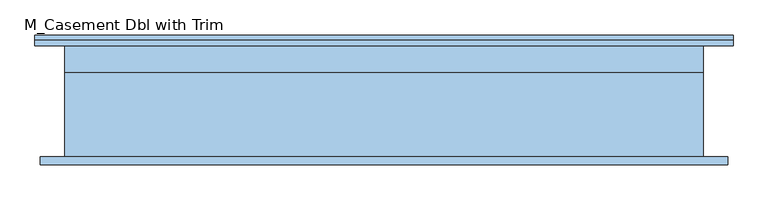
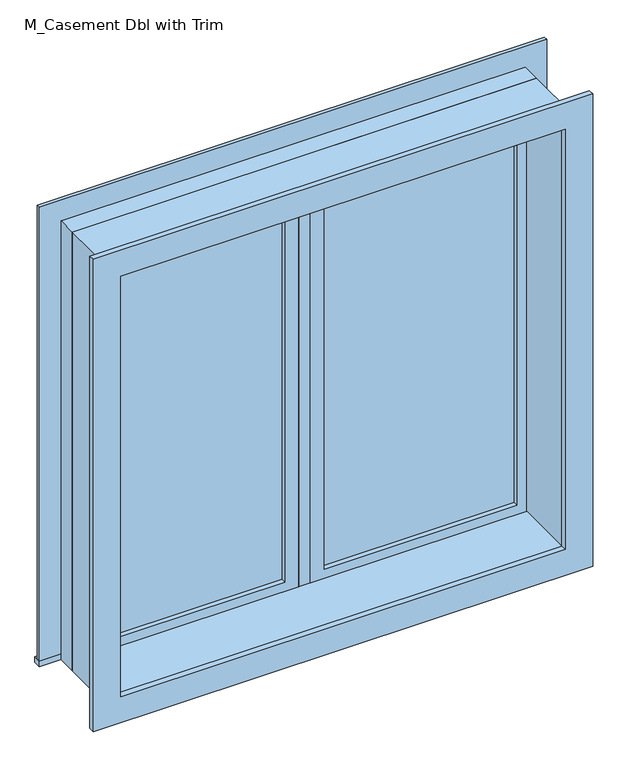
"""IFC4 building model written with IfcOpenShell, lengths in millimetres: window geometry, M_Casement Dbl with Trim : 150x150cm Pencere."""

from ifc_helpers import new_model, si_unit, frame, origin, place, context, project, spatial, polyline, outline, extrude, source, transform, mapped, element, save


def m_casement_dbl_with_trim_011da180(model_context):
    return source(origin(), model_context, "Body", "SweptSolid", [
        extrude(outline(polyline([(63.5, 114.175), (686.5, 114.175), (686.5, 101.475), (63.5, 101.475), (63.5, 114.175)])), frame((0.0, 0.0, 978.5), z_axis=(0.0, 0.0, 1.0), x_axis=(1.0, 0.0, 0.0)), (0.0, 0.0, 1.0), 1373.0),
        extrude(outline(polyline([(2395.95, 19.05), (934.05, 19.05), (934.05, 730.95), (2395.95, 730.95), (2395.95, 19.05)]), holes=[polyline([(2351.5, 63.5), (2351.5, 686.5), (978.5, 686.5), (978.5, 63.5), (2351.5, 63.5)])]), frame((0.0, 85.6, 0.0), z_axis=(0.0, 1.0, 0.0), x_axis=(0.0, 0.0, 1.0)), (0.0, 0.0, 1.0), 44.45),
        extrude(outline(polyline([(-819.95, 174.75), (819.95, 174.75), (819.95, 149.05), (-819.95, 149.05), (-819.95, 174.75)])), frame((0.0, 0.0, 915.0), z_axis=(0.0, 0.0, 1.0), x_axis=(1.0, 0.0, 0.0)), (0.0, 0.0, 1.0), 19.05),
        extrude(outline(polyline([(2395.95, -730.95), (2395.95, 730.95), (934.05, 730.95), (934.05, 819.95), (2484.95, 819.95), (2484.95, -819.95), (934.05, -819.95), (934.05, -730.95), (2395.95, -730.95)])), frame((0.0, 149.05, 0.0), z_axis=(0.0, 1.0, 0.0), x_axis=(0.0, 0.0, 1.0)), (0.0, 0.0, 1.0), 13.0),
        extrude(outline(polyline([(2472.25, 807.25), (2472.25, -807.25), (857.75, -807.25), (857.75, 807.25), (2472.25, 807.25)]), holes=[polyline([(2383.25, 718.25), (946.75, 718.25), (946.75, -718.25), (2383.25, -718.25), (2383.25, 718.25)])]), frame((0.0, -129.95, 0.0), z_axis=(0.0, 1.0, 0.0), x_axis=(0.0, 0.0, 1.0)), (0.0, 0.0, 1.0), 19.0),
        extrude(outline(polyline([(-63.5, 101.475), (-686.5, 101.475), (-686.5, 114.175), (-63.5, 114.175), (-63.5, 101.475)])), frame((0.0, 0.0, 978.5), z_axis=(0.0, 0.0, 1.0), x_axis=(1.0, 0.0, 0.0)), (0.0, 0.0, 1.0), 1373.0),
        extrude(outline(polyline([(2395.95, -730.95), (934.05, -730.95), (934.05, -19.05), (2395.95, -19.05), (2395.95, -730.95)]), holes=[polyline([(2351.5, -686.5), (2351.5, -63.5), (978.5, -63.5), (978.5, -686.5), (2351.5, -686.5)])]), frame((0.0, 85.6, 0.0), z_axis=(0.0, 1.0, 0.0), x_axis=(0.0, 0.0, 1.0)), (0.0, 0.0, 1.0), 44.45),
        extrude(outline(polyline([(2415.0, -750.0), (915.0, -750.0), (915.0, 750.0), (2415.0, 750.0), (2415.0, -750.0)]), holes=[polyline([(2383.25, -718.25), (2383.25, 718.25), (946.75, 718.25), (946.75, -718.25), (2383.25, -718.25)])]), frame((0.0, -110.95, 0.0), z_axis=(0.0, 1.0, 0.0), x_axis=(0.0, 0.0, 1.0)), (0.0, 0.0, 1.0), 196.55),
        extrude(outline(polyline([(2415.0, 750.0), (2415.0, -750.0), (915.0, -750.0), (915.0, 750.0), (2415.0, 750.0)]), holes=[polyline([(2395.95, 730.95), (934.05, 730.95), (934.05, -730.95), (2395.95, -730.95), (2395.95, 730.95)])]), frame((0.0, 85.6, 0.0), z_axis=(0.0, 1.0, 0.0), x_axis=(0.0, 0.0, 1.0)), (0.0, 0.0, 1.0), 63.45),
        extrude(outline(polyline([(19.05, 85.6), (-19.05, 85.6), (-19.05, 149.1), (19.05, 149.1), (19.05, 85.6)])), frame((0.0, 0.0, 934.05), z_axis=(0.0, 0.0, 1.0), x_axis=(1.0, 0.0, 0.0)), (0.0, 0.0, 1.0), 1461.9),
    ])


if __name__ == "__main__":
    model = new_model("IFC4")
    model_context = context("Model", 3, world=origin())
    ifc_project = project(units=[si_unit("LENGTHUNIT", "METRE", prefix="MILLI")], contexts=[model_context])
    site = spatial("IfcSite", under=ifc_project)
    building = spatial("IfcBuilding", under=site)
    placement = place(None, origin())
    m_casement_dbl_with_trim_shape = m_casement_dbl_with_trim_011da180(model_context)
    element("IfcWindow", 1, ObjectType="M_Casement Dbl with Trim : 150x150cm Pencere", at=placement, inside=building, context=model_context, shape_type="MappedRepresentation", body=[
        mapped(m_casement_dbl_with_trim_shape, transform((0.0, 0.0, 0.0), x_axis=(1.0, 0.0, 0.0), y_axis=(0.0, 1.0, 0.0), z_axis=(0.0, 0.0, 1.0))),
    ])
    save(model, "model.ifc")

# Revit data of these elements
# Type "M_Casement Dbl with Trim : 150x150cm Pencere"
#   Type Mark = "20"
#   Construction Type Id = "GSP4R"
#   Analytic Construction = "1/8 in Pilkington single glazing"
#   Visual Light Transmittance = 0.9
#   Solar Heat Gain Coefficient = 0.78
#   Heat Transfer Coefficient (U) = 3.6886 W/(m²·K)
#   Height = 150.00 cm
#   Default Sill Height = 91.50 cm
#   Trim Projection - Ext. = 1.30 cm
#   Trim Projection - Int. = 1.90 cm
#   Trim Width - Exterior = 8.90 cm
#   Trim Width - Interior = 8.90 cm
#   Width = 150.00 cm
#   Window Inset = 1.90 cm
#   Define Thermal Properties by = 1
#   Glass Pane Material = Glass
#   Sash = Sash
#   Trim Exterior Material = Trim
#   Trim Interior Material = Trim
#   Wall Closure = (empty or 0)
# Element 1 (IfcWindow, "M_Casement Dbl with Trim : 150x150cm Pencere")
#   Materials on its faces: "Trim", "Sash", "Glass"
# Materials
#   "Glass": class "Glass", colour RGB 0 128 192, transparency 0.9, Description = "Soda Lime Glass", Cost = 0
#   "Sash": class "Wood", colour RGB 224 178 126, transparency 0
#   "Trim": class "Wood", colour RGB 224 178 126, transparency 0
